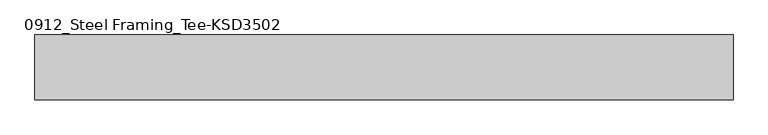
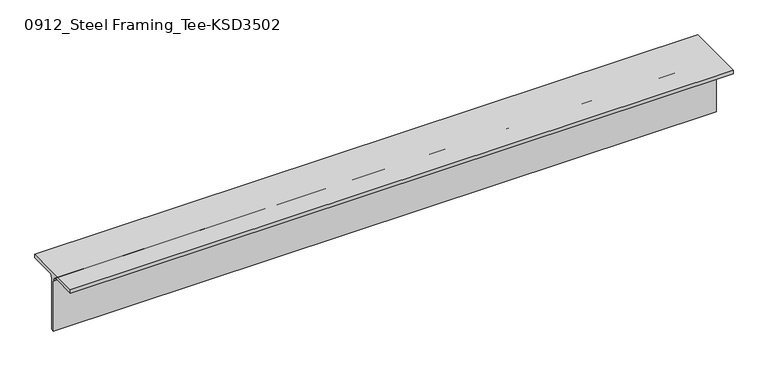
"""IFC4 building model written with IfcOpenShell, lengths in millimetres: member geometry, 0912_Steel Framing_Tee-KSD3502 : H_SB_ASB_CT-150x150x6.5x9."""

from ifc_helpers import new_model, si_unit, point, frame, frame_2d, origin, place, context, project, spatial, polyline, circle_curve, trimmed, segment, composite_curve, outline, extrude, source, transform, mapped, element, save


def member_0912_steel_framing_tee_ksd3502_413dd121(model_context):
    return source(origin(), model_context, "Body", "SweptSolid", [
        extrude(outline(composite_curve([segment(polyline([(75.0, 75.0), (75.0, 66.0), (16.25, 66.0)]), True, "CONTINUOUS"), segment(trimmed(circle_curve(frame_2d((16.25, 53.0)), 13.0), [point((16.25, 66.0))], [point((3.25, 53.0))], True, "CARTESIAN"), True, "CONTINUOUS"), segment(polyline([(3.25, 53.0), (3.25, -75.0), (-3.25, -75.0), (-3.25, 53.0)]), True, "CONTINUOUS"), segment(trimmed(circle_curve(frame_2d((-16.25, 53.0)), 13.0), [point((-3.25, 53.0))], [point((-16.25, 66.0))], True, "CARTESIAN"), True, "CONTINUOUS"), segment(polyline([(-16.25, 66.0), (-75.0, 66.0), (-75.0, 75.0), (75.0, 75.0)]), True, "CONTINUOUS")], self_intersect=False)), frame((-807.1, 0.0, 0.0), z_axis=(1.0, 0.0, 0.0), x_axis=(0.0, 1.0, 0.0)), (0.0, 0.0, 1.0), 1614.2),
    ])


if __name__ == "__main__":
    model = new_model("IFC4")
    model_context = context("Model", 3, world=origin())
    ifc_project = project(units=[si_unit("LENGTHUNIT", "METRE", prefix="MILLI")], contexts=[model_context])
    site = spatial("IfcSite", under=ifc_project)
    building = spatial("IfcBuilding", under=site)
    placement = place(None, origin())
    member_0912_steel_framing_tee_ksd3502_shape = member_0912_steel_framing_tee_ksd3502_413dd121(model_context)
    element("IfcMember", 1, ObjectType="0912_Steel Framing_Tee-KSD3502 : H_SB_ASB_CT-150x150x6.5x9", at=placement, inside=building, context=model_context, shape_type="MappedRepresentation", body=[
        mapped(member_0912_steel_framing_tee_ksd3502_shape, transform((0.0, 0.0, 0.0), x_axis=(1.0, 0.0, 0.0), y_axis=(0.0, 1.0, 0.0), z_axis=(0.0, 0.0, 1.0))),
    ])
    save(model, "model.ifc")

# Revit data of these elements
# Type "0912_Steel Framing_Tee-KSD3502 : H_SB_ASB_CT-150x150x6.5x9"
#   H_WM Code_1 = "S01AA003-00001 | Main Steel Structure Fabrication Work | Shelter/Building | Light Steel - Standard (30KG/M>Weight) | Material: (   )"
#   H_WM Code_2 = "S03AA029-00001 | Main Steel Structure Erection Work | Shelter/Building | Light Steel (30KG/M>Weight) | Material: (   )"
#   H_WM Code_3 = "S01AA010-00001 | Main Steel Structure Fabrication Work | Shelter/Building | Steel Painting/Coating | for Non-Fireproofed Steel Surface, Surface Preparation, Primer, Second & Final Coat | Material: (   )"
#   H_Q'ty Cal Type Tag = "SB-Q2"
#   Width = 15.0 cm
#   Web Thickness = 0.65 cm
#   Web Fillet = 1.3 cm
#   Section Area = 23.39 cm²
#   Perimeter = 0.60 m²/m
#   Nominal Weight = 18.40 kgf/m
#   Height = 15.0 cm
#   Flange Thickness = 0.9 cm
#   Centroid Vertical = 7.5 cm
#   Centroid Horizontal = 7.5 cm
#   Length [instance default] = 1.5000 m
#   Structural Material [instance default] = Steel, 45-345
#   Warping Constant = (empty or 0)
#   Torsional Moment of Inertia = 0
#   Section Name Key = ""
#   Plastic Modulus weak axis = 0
#   Plastic Modulus strong axis = 0
#   Moment of Inertia weak axis = 0
#   Moment of Inertia strong axis = 0
#   Elastic Modulus weak axis = 0
#   Elastic Modulus strong axis = 0
#   Bolt Spacing = 0
#   Assembly Code = ""
# Element 1 (IfcMember, "0912_Steel Framing_Tee-KSD3502 : H_SB_ASB_CT-150x150x6.5x9")
#   Structural Material = none
# Materials
#   "Steel, 45-345": class "Metal", colour RGB 189 187 185, transparency 0, Description = "Steel 345 MPa", Cost = 0
